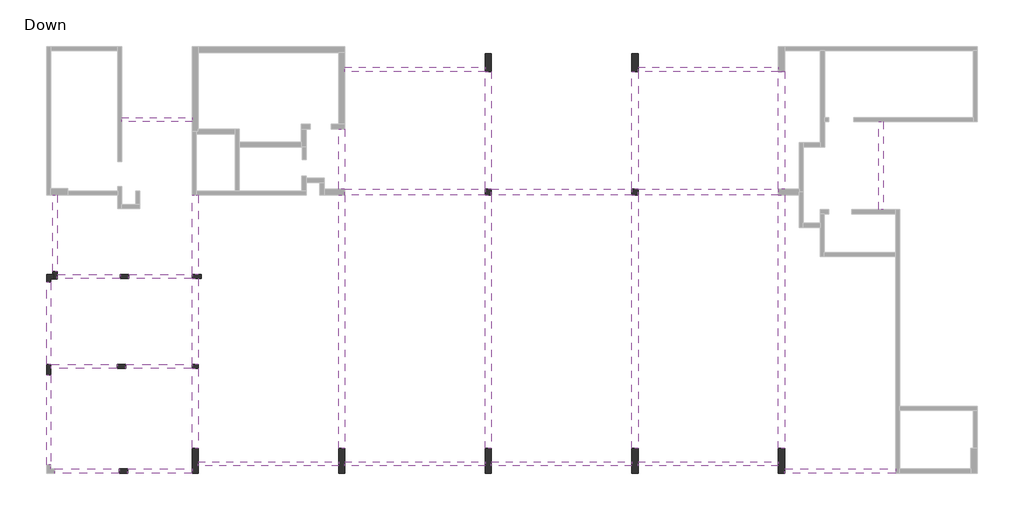
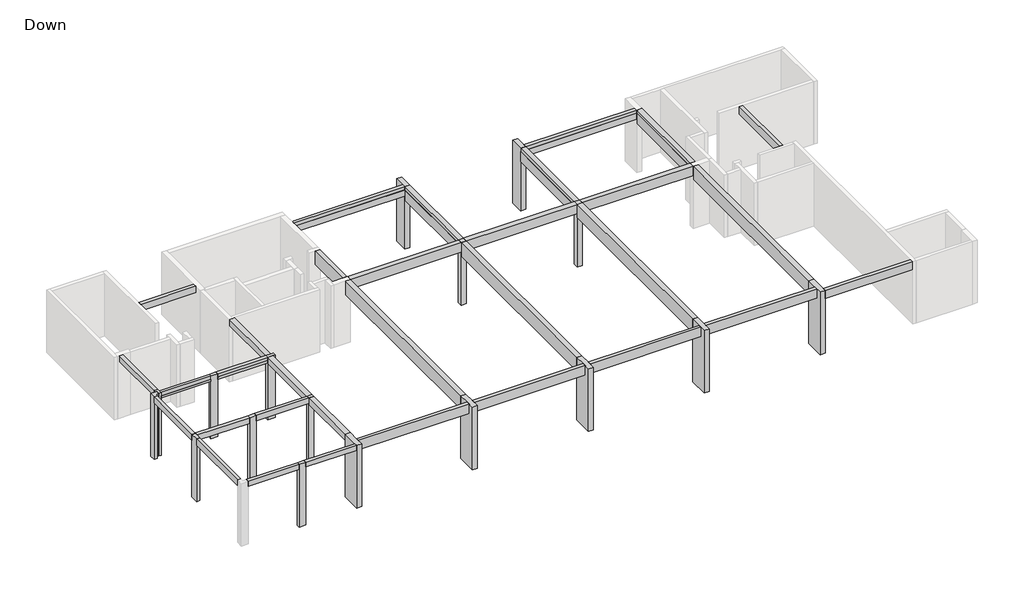
# One storey, part 2 of 2: 32 beams, 17 columns.
# Revit data of these elements (continued)
# Element 41 (IfcColumn, "Concrete Rectengular Column : 30/120") (continued)
#   Materials on its faces: "Concrete"
# Element 42 (IfcColumn, "Concrete Rectengular Column : 30/120")
#   Comments = ""
#   Mark = "C10"
#   SOFiSTiK_AMG_Comments = ""
#   SOFiSTiK_AMG_Scheduled = yes
#   SOFiSTiK_AMG_Adjusted = yes
#   Structural Material = Concrete
#   Phase Created = New Construction
#   Materials on its faces: "Concrete"
# Element 43 (IfcColumn, "Concrete Rectengular Column : 30/120")
#   Comments = ""
#   Mark = "C11"
#   SOFiSTiK_AMG_Comments = ""
#   SOFiSTiK_AMG_Scheduled = yes
#   SOFiSTiK_AMG_Adjusted = yes
#   Structural Material = Concrete
#   Phase Created = New Construction
#   Materials on its faces: "Concrete"
# Element 44 (IfcColumn, "Concrete Rectengular Column : 30/30")
#   Comments = ""
#   Mark = "C12"
#   SOFiSTiK_AMG_Comments = ""
#   SOFiSTiK_AMG_Scheduled = yes
#   SOFiSTiK_AMG_Adjusted = yes
#   Structural Material = Concrete
#   Phase Created = New Construction
#   Materials on its faces: "Concrete"
# Element 45 (IfcColumn, "Concrete Rectengular Column : 30/30")
#   Comments = ""
#   Mark = "C13"
#   SOFiSTiK_AMG_Comments = ""
#   SOFiSTiK_AMG_Scheduled = yes
#   SOFiSTiK_AMG_Adjusted = yes
#   Structural Material = Concrete
#   Phase Created = New Construction
#   Materials on its faces: "Concrete"
# Element 46 (IfcColumn, "Concrete Rectengular Column : 30/85")
#   Comments = ""
#   Mark = "C14"
#   SOFiSTiK_AMG_Comments = ""
#   SOFiSTiK_AMG_Scheduled = yes
#   SOFiSTiK_AMG_Adjusted = yes
#   Structural Material = Concrete
#   Phase Created = New Construction
#   Materials on its faces: "Concrete"
# Element 47 (IfcColumn, "Concrete Rectengular Column : 30/85")
#   Comments = ""
#   Mark = "C15"
#   SOFiSTiK_AMG_Comments = ""
#   SOFiSTiK_AMG_Scheduled = yes
#   SOFiSTiK_AMG_Adjusted = yes
#   Structural Material = Concrete
#   Phase Created = New Construction
#   Materials on its faces: "Concrete"
# Element 48 (IfcColumn, "L Column : 35/35/20/20")
#   Comments = ""
#   Mark = "C16"
#   SOFiSTiK_AMG_Comments = ""
#   SOFiSTiK_AMG_Scheduled = yes
#   SOFiSTiK_AMG_Adjusted = yes
#   Structural Material = Concrete
#   Phase Created = New Construction
# Element 49 (IfcColumn, "L Column : 35/35/20/20")
#   Comments = ""
#   Mark = "C17"
#   SOFiSTiK_AMG_Comments = ""
#   SOFiSTiK_AMG_Scheduled = yes
#   SOFiSTiK_AMG_Adjusted = yes
#   Structural Material = Concrete
#   Phase Created = New Construction
# Materials
#   "Concrete": class "Concrete", colour RGB 192 192 192, transparency 0, Keynote = "01000", Description = "Cast-in-place concrete", Cost = 0
#   "Concrete, Cast-in-Place gray": class "Concrete", colour RGB 192 192 192, transparency 0, Description = "Cast-in-place concrete", Cost = 0
